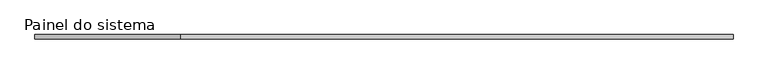
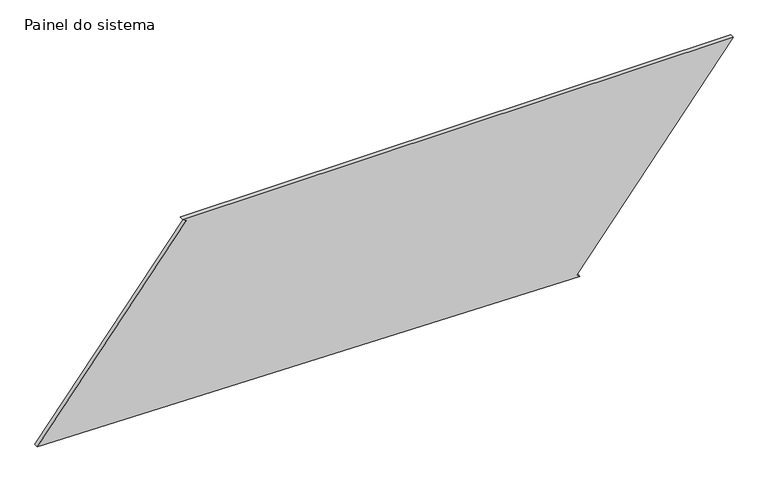
"""IFC4 building model written with IfcOpenShell, lengths in millimetres: plate geometry, Painel do sistema : Envidraçado."""

from ifc_helpers import new_model, si_unit, frame, origin, place, context, project, spatial, polyline, outline, extrude, source, transform, mapped, element, save


def painel_do_sistema_2c199968(model_context):
    return source(origin(), model_context, "Body", "SweptSolid", [
        extrude(outline(polyline([(0.0, 1151.7694678), (15.5601026, 1132.2020662), (1178.9718271, 2057.3533031), (1178.9718271, -1197.5869624), (1163.4117245, -1178.0195608), (57.6171855, -2057.3533031), (0.0, 1151.7694678)])), frame((0.0, 24.5, 0.0), z_axis=(0.0, 1.0, 0.0), x_axis=(0.0, 0.0, 1.0)), (0.0, 0.0, 1.0), 25.0),
    ])


if __name__ == "__main__":
    model = new_model("IFC4")
    model_context = context("Model", 3, world=origin())
    ifc_project = project(units=[si_unit("LENGTHUNIT", "METRE", prefix="MILLI")], contexts=[model_context])
    site = spatial("IfcSite", under=ifc_project)
    building = spatial("IfcBuilding", under=site)
    placement = place(None, origin())
    painel_do_sistema_shape = painel_do_sistema_2c199968(model_context)
    element("IfcPlate", 1, ObjectType="Painel do sistema : Envidraçado", at=placement, inside=building, context=model_context, shape_type="MappedRepresentation", body=[
        mapped(painel_do_sistema_shape, transform((0.0, 0.0, 0.0), x_axis=(1.0, 0.0, 0.0), y_axis=(0.0, 1.0, 0.0), z_axis=(0.0, 0.0, 1.0))),
    ])
    save(model, "model.ifc")

# Revit data of these elements
# Type "Painel do sistema : Envidraçado"
#   Construction Type Id = "GSP4R"
#   Analytic Construction = "Vidraça única Pilkington 1/8 pol"
#   Visual Light Transmittance = 0.9
#   Solar Heat Gain Coefficient = 0.86
#   Heat Transfer Coefficient (U) = 6.7069 W/(m²·K)
# Element 1 (IfcPlate, "Painel do sistema : Envidraçado")
#   Materials on its faces: "Vidro"
# Materials
#   "Vidro": class "Vidro", colour RGB 0 128 192, transparency 0.9, Description = "Vidro de sílica", Cost = 0
